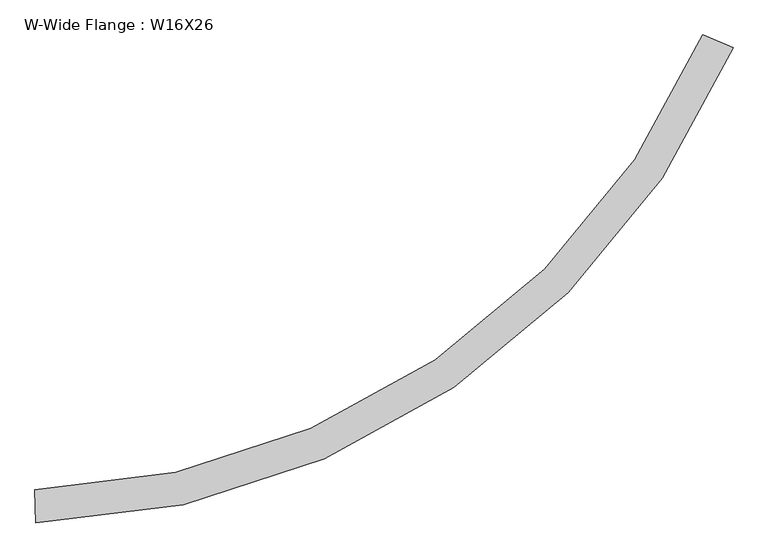
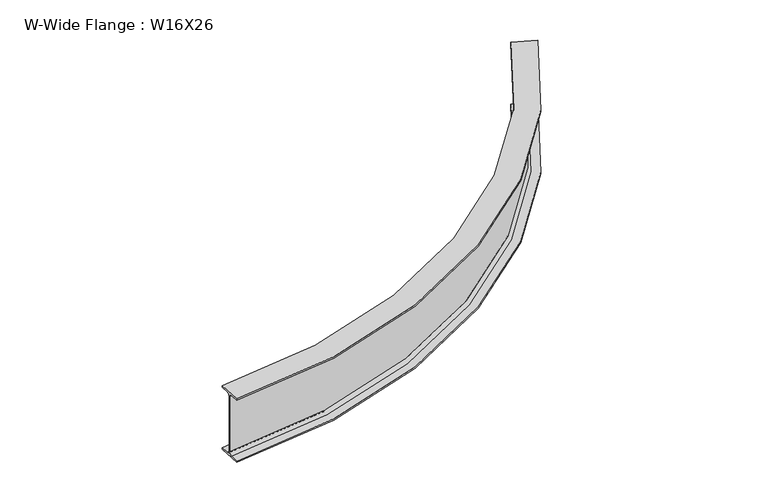
"""IFC4 building model written with IfcOpenShell, lengths in millimetres: beam geometry, W-Wide Flange : W16X26."""

from ifc_helpers import new_model, si_unit, point, frame, origin, place, context, project, spatial, polyline, circle_curve, ellipse_curve, trimmed, source, transform, mapped, element, save
from ifc_brep_helpers import plane_surface, cylinder_surface, revolved_surface, advanced_brep


def w_wide_flange_w16x26_f95649ea(model_context):
    return source(origin(), model_context, "Body", "AdvancedBrep", [
        advanced_brep(
        [(3047.7966024, 1943.1127488, -190.5496094), (3047.7966024, 1943.1127488, -199.2808594), (2919.3102414, 1997.9520143, -199.2808594), (2919.3102414, 1997.9520143, -190.5496094), (2963.842446, 1978.9452234, -190.5496094), (2980.6332773, 1971.7787285, -172.2933594), (2980.6332773, 1971.7787285, 172.2933594), (2963.842446, 1978.9452234, 190.5496094), (2919.3102414, 1997.9520143, 190.5496094), (2919.3102414, 1997.9520143, 199.2808594), (3047.7966024, 1943.1127488, 199.2808594), (3047.7966024, 1943.1127488, 190.5496094), (3003.2643977, 1962.1195397, 190.5496094), (2986.4735664, 1969.2860346, 172.2933594), (2986.4735664, 1969.2860346, -172.2933594), (3003.2643977, 1962.1195397, -190.5496094), (98.9962567, -68.3709627, -190.5496094), (97.5497949, -19.9738233, -190.5496094), (97.0044076, -1.7257216, -172.2933594), (97.0044076, -1.7257216, 172.2933594), (97.5497949, -19.9738233, 190.5496094), (98.9962567, -68.3709627, 190.5496094), (98.9962567, -68.3709627, 199.2808594), (94.8228586, 71.2666853, 199.2808594), (94.8228586, 71.2666853, 190.5496094), (96.2693204, 22.8695459, 190.5496094), (96.8147077, 4.6214442, 172.2933594), (96.8147077, 4.6214442, -172.2933594), (96.2693204, 22.8695459, -190.5496094), (94.8228586, 71.2666853, -190.5496094), (94.8228586, 71.2666853, -199.2808594), (98.9962567, -68.3709627, -199.2808594)],
        [
            (0, 1),
            (1, 2),
            (2, 3),
            (3, 4),
            (4, 5, circle_curve(frame((2963.842446, 1978.9452234, -172.2933594), z_axis=(-0.3925502179509604, -0.9197305727149955, 0.0), x_axis=(-0.9197305727149955, 0.3925502179509604, 0.0)), 18.25625)),
            (5, 6),
            (6, 7, circle_curve(frame((2963.842446, 1978.9452234, 172.2933594), z_axis=(-0.3925502179509604, -0.9197305727149955, 0.0), x_axis=(-0.9197305727149955, 0.3925502179509604, 0.0)), 18.25625)),
            (7, 8),
            (8, 9),
            (9, 10),
            (10, 11),
            (11, 12),
            (12, 13, circle_curve(frame((3003.2643977, 1962.1195397, 172.2933594), z_axis=(-0.3925502179509604, -0.9197305727149955, 0.0), x_axis=(-0.9197305727149955, 0.3925502179509604, 0.0)), 18.25625)),
            (13, 14),
            (14, 15, circle_curve(frame((3003.2643977, 1962.1195397, -172.2933594), z_axis=(-0.3925502179509604, -0.9197305727149955, 0.0), x_axis=(-0.9197305727149955, 0.3925502179509604, 0.0)), 18.25625)),
            (15, 0),
            (16, 17),
            (17, 18, circle_curve(frame((97.5497949, -19.9738233, -172.2933594), z_axis=(0.99955367237749, 0.029874002689184272, 0.0), x_axis=(-0.029874002689184272, 0.99955367237749, 0.0)), 18.25625)),
            (18, 19),
            (19, 20, circle_curve(frame((97.5497949, -19.9738233, 172.2933594), z_axis=(0.99955367237749, 0.029874002689184272, 0.0), x_axis=(-0.029874002689184272, 0.99955367237749, 0.0)), 18.25625)),
            (20, 21),
            (21, 22),
            (22, 23),
            (23, 24),
            (24, 25),
            (25, 26, circle_curve(frame((96.2693204, 22.8695459, 172.2933594), z_axis=(0.99955367237749, 0.029874002689184272, 0.0), x_axis=(-0.029874002689184272, 0.99955367237749, 0.0)), 18.25625)),
            (26, 27),
            (27, 28, circle_curve(frame((96.2693204, 22.8695459, -172.2933594), z_axis=(0.99955367237749, 0.029874002689184272, 0.0), x_axis=(-0.029874002689184272, 0.99955367237749, 0.0)), 18.25625)),
            (28, 29),
            (29, 30),
            (30, 31),
            (31, 16),
            (15, 17, circle_curve(frame((0.0, 3243.9428571, -190.5496094), z_axis=(0.0, 0.0, -1.0), x_axis=(-1.0, 0.0, 0.0)), 3265.3741071)),
            (16, 0, circle_curve(frame((0.0, 3243.9428571, -190.5496094), z_axis=(0.0, 0.0, 1.0), x_axis=(-1.0, 0.0, 0.0)), 3313.7928571)),
            (14, 18, circle_curve(frame((0.0, 3243.9428571, -172.2933594), z_axis=(0.0, 0.0, -1.0), x_axis=(-1.0, 0.0, 0.0)), 3247.1178571)),
            (13, 19, circle_curve(frame((0.0, 3243.9428571, 172.2933594), z_axis=(0.0, 0.0, -1.0), x_axis=(-1.0, 0.0, 0.0)), 3247.1178571)),
            (12, 20, circle_curve(frame((0.0, 3243.9428571, 190.5496094), z_axis=(0.0, 0.0, -1.0), x_axis=(-1.0, 0.0, 0.0)), 3265.3741071)),
            (11, 21, circle_curve(frame((0.0, 3243.9428571, 190.5496094), z_axis=(0.0, 0.0, -1.0), x_axis=(-1.0, 0.0, 0.0)), 3313.7928571)),
            (10, 22, circle_curve(frame((0.0, 3243.9428571, 199.2808594), z_axis=(0.0, 0.0, -1.0), x_axis=(-1.0, 0.0, 0.0)), 3313.7928571)),
            (9, 23, circle_curve(frame((0.0, 3243.9428571, 199.2808594), z_axis=(0.0, 0.0, -1.0), x_axis=(-1.0, 0.0, 0.0)), 3174.0928571)),
            (8, 24, circle_curve(frame((0.0, 3243.9428571, 190.5496094), z_axis=(0.0, 0.0, -1.0), x_axis=(-1.0, 0.0, 0.0)), 3174.0928571)),
            (7, 25, circle_curve(frame((0.0, 3243.9428571, 190.5496094), z_axis=(0.0, 0.0, -1.0), x_axis=(-1.0, 0.0, 0.0)), 3222.5116071)),
            (6, 26, circle_curve(frame((0.0, 3243.9428571, 172.2933594), z_axis=(0.0, 0.0, -1.0), x_axis=(-1.0, 0.0, 0.0)), 3240.7678571)),
            (5, 27, circle_curve(frame((0.0, 3243.9428571, -172.2933594), z_axis=(0.0, 0.0, -1.0), x_axis=(-1.0, 0.0, 0.0)), 3240.7678571)),
            (4, 28, circle_curve(frame((0.0, 3243.9428571, -190.5496094), z_axis=(0.0, 0.0, -1.0), x_axis=(-1.0, 0.0, 0.0)), 3222.5116071)),
            (3, 29, circle_curve(frame((0.0, 3243.9428571, -190.5496094), z_axis=(0.0, 0.0, -1.0), x_axis=(-1.0, 0.0, 0.0)), 3174.0928571)),
            (2, 30, circle_curve(frame((0.0, 3243.9428571, -199.2808594), z_axis=(0.0, 0.0, -1.0), x_axis=(-1.0, 0.0, 0.0)), 3174.0928571)),
            (1, 31, circle_curve(frame((0.0, 3243.9428571, -199.2808594), z_axis=(0.0, 0.0, -1.0), x_axis=(-1.0, 0.0, 0.0)), 3313.7928571)),
        ],
        [
            plane_surface(frame((2983.5534219, 1970.5323816, 0.0), z_axis=(0.39255021795095457, 0.9197305727149979, 0.0), x_axis=(0.0, 0.0, 1.0))),
            plane_surface(frame((96.9095576, 1.4478613, 0.0), z_axis=(-0.9995536723774898, -0.029874002689190826, 0.0), x_axis=(0.0, 0.0, 1.0))),
            plane_surface(frame((0.0, 3243.9428571, -190.5496094), z_axis=(0.0, 0.0, 1.0), x_axis=(-1.0, 0.0, 0.0))),
            revolved_surface(trimmed(ellipse_curve(frame((-3265.3741071, 3243.9428571, -172.2933594), z_axis=(0.0, 1.0, 0.0), x_axis=(1.0, 0.0, 0.0)), 18.25625, 18.25625), [point((-3247.1178571, 3243.9428571, -172.2933594))], [point((-3265.3741071, 3243.9428571, -190.5496094))], True, "CARTESIAN"), (0.0, 3243.9428571, 0.0), (0.0, 0.0, -1.0)),
            cylinder_surface(frame((0.0, 3243.9428571, 0.0), z_axis=(0.0, 0.0, -1.0), x_axis=(-1.0, 0.0, 0.0)), 3247.1178571),
            revolved_surface(trimmed(ellipse_curve(frame((-3265.3741071, 3243.9428571, 172.2933594), z_axis=(0.0, 1.0, 0.0), x_axis=(1.0, 0.0, 0.0)), 18.25625, 18.25625), [point((-3265.3741071, 3243.9428571, 190.5496094))], [point((-3247.1178571, 3243.9428571, 172.2933594))], True, "CARTESIAN"), (0.0, 3243.9428571, 0.0), (0.0, 0.0, -1.0)),
            plane_surface(frame((0.0, 3243.9428571, 190.5496094), z_axis=(0.0, 0.0, -1.0), x_axis=(-1.0, 0.0, 0.0))),
            cylinder_surface(frame((0.0, 3243.9428571, 0.0), z_axis=(0.0, 0.0, -1.0), x_axis=(-1.0, 0.0, 0.0)), 3313.7928571),
            plane_surface(frame((0.0, 3243.9428571, 199.2808594), z_axis=(0.0, 0.0, 1.0), x_axis=(-1.0, 0.0, 0.0))),
            revolved_surface(polyline([(-3174.0928571, 3243.9428571, 190.5496094), (-3174.0928571, 3243.9428571, 199.2808594)]), (0.0, 3243.9428571, 0.0), (0.0, 0.0, -1.0)),
            revolved_surface(trimmed(ellipse_curve(frame((-3222.5116071, 3243.9428571, 172.2933594), z_axis=(0.0, 1.0, 0.0), x_axis=(1.0, 0.0, 0.0)), 18.25625, 18.25625), [point((-3240.7678571, 3243.9428571, 172.2933594))], [point((-3222.5116071, 3243.9428571, 190.5496094))], True, "CARTESIAN"), (0.0, 3243.9428571, 0.0), (0.0, 0.0, -1.0)),
            revolved_surface(polyline([(-3240.7678571, 3243.9428571, -172.2933594), (-3240.7678571, 3243.9428571, 172.2933594)]), (0.0, 3243.9428571, 0.0), (0.0, 0.0, -1.0)),
            revolved_surface(trimmed(ellipse_curve(frame((-3222.5116071, 3243.9428571, -172.2933594), z_axis=(0.0, 1.0, 0.0), x_axis=(1.0, 0.0, 0.0)), 18.25625, 18.25625), [point((-3222.5116071, 3243.9428571, -190.5496094))], [point((-3240.7678571, 3243.9428571, -172.2933594))], True, "CARTESIAN"), (0.0, 3243.9428571, 0.0), (0.0, 0.0, -1.0)),
            revolved_surface(polyline([(-3174.0928571, 3243.9428571, -199.2808594), (-3174.0928571, 3243.9428571, -190.5496094)]), (0.0, 3243.9428571, 0.0), (0.0, 0.0, -1.0)),
            plane_surface(frame((0.0, 3243.9428571, -199.2808594), z_axis=(0.0, 0.0, -1.0), x_axis=(-1.0, 0.0, 0.0))),
        ],
        [
            (0, [[1, 2, 3, 4, 5, 6, 7, 8, 9, 10, 11, 12, 13, 14, 15, 16]]),
            (1, [[17, 18, 19, 20, 21, 22, 23, 24, 25, 26, 27, 28, 29, 30, 31, 32]]),
            (2, [[33, -17, 34, -16]]),
            (3, [[35, -18, -33, -15]]),
            (4, [[36, -19, -35, -14]]),
            (5, [[37, -20, -36, -13]]),
            (6, [[38, -21, -37, -12]]),
            (7, [[39, -22, -38, -11]]),
            (8, [[40, -23, -39, -10]]),
            (9, [[41, -24, -40, -9]]),
            (6, [[42, -25, -41, -8]]),
            (10, [[43, -26, -42, -7]]),
            (11, [[44, -27, -43, -6]]),
            (12, [[45, -28, -44, -5]]),
            (2, [[46, -29, -45, -4]]),
            (13, [[47, -30, -46, -3]]),
            (14, [[48, -31, -47, -2]]),
            (7, [[-34, -32, -48, -1]]),
        ],
    ),
    ])


if __name__ == "__main__":
    model = new_model("IFC4")
    model_context = context("Model", 3, world=origin())
    ifc_project = project(units=[si_unit("LENGTHUNIT", "METRE", prefix="MILLI")], contexts=[model_context])
    site = spatial("IfcSite", under=ifc_project)
    building = spatial("IfcBuilding", under=site)
    placement = place(None, origin())
    w_wide_flange_w16x26_shape = w_wide_flange_w16x26_f95649ea(model_context)
    element("IfcBeam", 1, ObjectType="W-Wide Flange : W16X26", at=placement, inside=building, context=model_context, shape_type="MappedRepresentation", body=[
        mapped(w_wide_flange_w16x26_shape, transform((0.0, 0.0, 0.0), x_axis=(1.0, 0.0, 0.0), y_axis=(0.0, 1.0, 0.0), z_axis=(0.0, 0.0, 1.0))),
    ])
    save(model, "model.ifc")

# Revit data of these elements
# Type "W-Wide Flange : W16X26"
#   Assembly Code = "B10"
#   W = 26
#   Start Extension Calculation [instance default] = 10' - 0"
#   Start Extension [instance default] = -0' - 0 1/2"
#   End Extension Calculation [instance default] = 10' - 0"
#   End Extension [instance default] = -0' - 0 1/2"
#   Length [instance default] = 5' - 0"
#   bf = 0' - 5 1/2"
#   d = 1' - 3 177/256"
#   k = 0' - 1 1/16"
#   k2 = 0' - 0 23/32"
#   tf = 0' - 0 11/32"
#   tw = 0' - 0 1/4"
#   A = 0.05 SF
#   Beam Material [instance default] = Metal - Steel - ASTM A992
# Element 1 (IfcBeam, "W-Wide Flange : W16X26")
#   Materials on its faces: "Metal - Steel - ASTM A992"
# Materials
#   "Metal - Steel - ASTM A992": class "Metal", colour RGB 128 0 0, transparency 0
